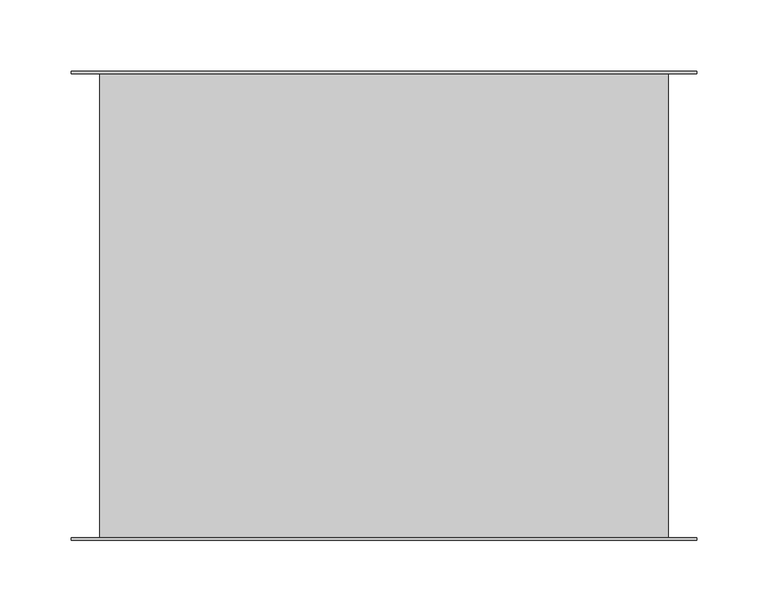
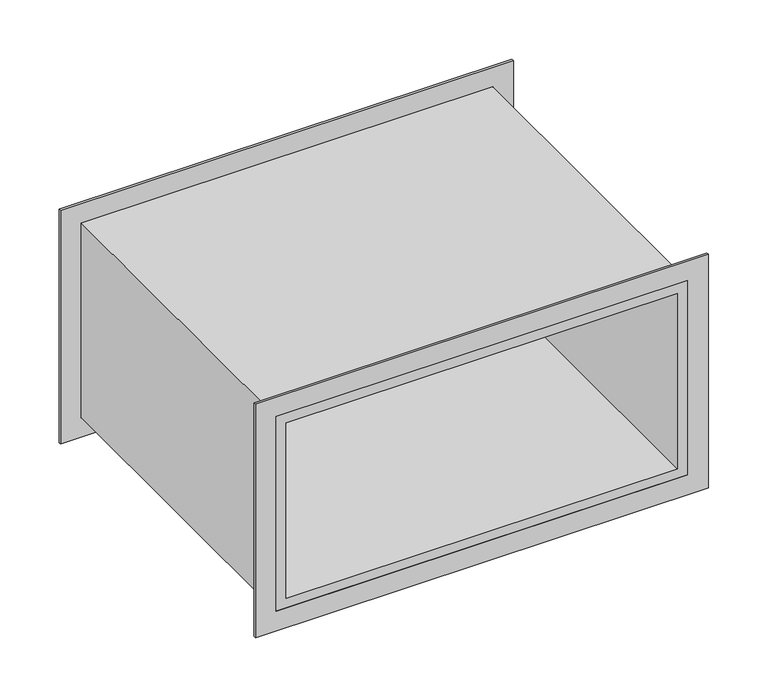
"""IFC4 building model written with IfcOpenShell, lengths in millimetres: proxy geometry, Фильтр карманный DFKRU : DFKRU 40-20."""

from ifc_helpers import new_model, si_unit, frame, origin, place, context, project, spatial, polyline, outline, extrude, source, transform, mapped, element, save


def mechanical_equipment_834d7efa(model_context):
    return source(origin(), model_context, "Body", "SweptSolid", [
        extrude(outline(polyline([(120.0, 220.0), (120.0, -220.0), (-120.0, -220.0), (-120.0, 220.0), (120.0, 220.0)]), holes=[polyline([(-100.0, 200.0), (-100.0, -200.0), (100.0, -200.0), (100.0, 200.0), (-100.0, 200.0)])]), frame((0.0, 163.0, 0.0), z_axis=(0.0, 1.0, 0.0), x_axis=(0.0, 0.0, 1.0)), (0.0, 0.0, 1.0), 2.0),
        extrude(outline(polyline([(120.0, -220.0), (-120.0, -220.0), (-120.0, 220.0), (120.0, 220.0), (120.0, -220.0)]), holes=[polyline([(100.0, 200.0), (-100.0, 200.0), (-100.0, -200.0), (100.0, -200.0), (100.0, 200.0)])]), frame((0.0, -165.0, 0.0), z_axis=(0.0, 1.0, 0.0), x_axis=(0.0, 0.0, 1.0)), (0.0, 0.0, 1.0), 2.0),
        extrude(outline(polyline([(100.0, 200.0), (100.0, -200.0), (-100.0, -200.0), (-100.0, 200.0), (100.0, 200.0)]), holes=[polyline([(90.0, 190.0), (-90.0, 190.0), (-90.0, -190.0), (90.0, -190.0), (90.0, 190.0)])]), frame((0.0, -165.0, 0.0), z_axis=(0.0, 1.0, 0.0), x_axis=(0.0, 0.0, 1.0)), (0.0, 0.0, 1.0), 330.0),
    ])


if __name__ == "__main__":
    model = new_model("IFC4")
    model_context = context("Model", 3, world=origin())
    ifc_project = project(units=[si_unit("LENGTHUNIT", "METRE", prefix="MILLI")], contexts=[model_context])
    site = spatial("IfcSite", under=ifc_project)
    building = spatial("IfcBuilding", under=site)
    placement = place(None, origin())
    mechanical_equipment_shape = mechanical_equipment_834d7efa(model_context)
    element("IfcBuildingElementProxy", 1, Name="Фильтр карманный DFKRU : DFKRU 40-20", ObjectType="Фильтр карманный DFKRU : DFKRU 40-20", at=placement, inside=building, context=model_context, shape_type="MappedRepresentation", body=[
        mapped(mechanical_equipment_shape, transform((0.0, 0.0, 0.0), x_axis=(1.0, 0.0, 0.0), y_axis=(0.0, 1.0, 0.0), z_axis=(0.0, 0.0, 1.0))),
    ])
    save(model, "model.ifc")

# Revit data of these elements
# Type "Фильтр карманный DFKRU : DFKRU 40-20"
#   Manufacturer = "WAER"
#   URL = "https://waer-air.com/"
#   ADSK_Система_Имя [instance default] = ""
#   ADSK_Наименование краткое = "DFKRU 40-20"
#   ADSK_Наименование = "Фильтр карманный укороченный DFKRU 40-20"
#   ADSK_Масса_Текст = "6.8"
#   ADSK_Марка = ""
#   ADSK_Код изделия = ""
#   ADSK_Завод-изготовитель = "WAER"
#   ADSK_Единица измерения = "шт."
#   ADSK_Расход воздуха = 0 m³/h
#   ADSK_Размер_Ширина = 400 mm
#   ADSK_Размер_Длина = 330 mm
#   ADSK_Размер_Высота = 200 mm
#   ADSK_Потеря давления воздуха = 0.0 Pa
#   ADSK_Масса = 6.8
#   ADSK_Количество = 1
#   ADSK_Фильтрующая вставка = element 1323802
#   Default Elevation = 0
#   Keynote = ""
